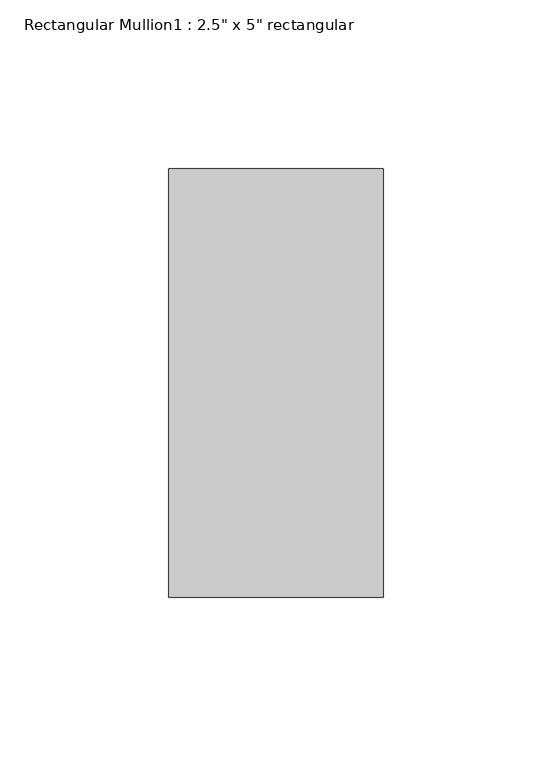
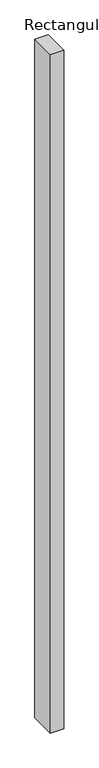
"""IFC4 building model written with IfcOpenShell, lengths in millimetres: member geometry."""

import ifcopenshell
import ifcopenshell.guid

model = None  # the IFC model being written
_history = None  # IfcOwnerHistory: only IFC2X3 demands one
_inside = {}  # id of a spatial element -> (the spatial element, [elements in it])
_under = {}  # id of a project, library or spatial element -> (it, [spatial elements below it])
_declared = {}  # id of a project -> (the project, [libraries it declares])
_typed = {}  # id of a type object -> (the type object, [elements of that type])
_made_of = {}  # id of a material, layer set ... -> (it, [elements and type objects made of it])


def new_model(schema):
    """Start an empty IFC model of exactly this schema.

    Asked for "IFC4X3", IfcOpenShell would pick the latest addendum, in which some entities
    have other attributes; the version numbers below select the first issue.
    IFC2X3 requires an IfcOwnerHistory on every rooted entity: one is made here for all.
    """
    global model, _history
    if schema == "IFC4X3":
        model = ifcopenshell.file(schema_version=(4, 3, 0, 0))
    else:
        model = ifcopenshell.file(schema=schema)
    _inside.clear()
    _under.clear()
    _declared.clear()
    _typed.clear()
    _made_of.clear()
    _history = None
    if model.schema == "IFC2X3":
        org = make("IfcOrganization", Name="unknown")
        user = make(
            "IfcPersonAndOrganization",
            ThePerson=make("IfcPerson", FamilyName="unknown"),
            TheOrganization=org,
        )
        app = make(
            "IfcApplication",
            ApplicationDeveloper=org,
            Version="unknown",
            ApplicationFullName="unknown",
            ApplicationIdentifier="unknown",
        )
        _history = make(
            "IfcOwnerHistory",
            OwningUser=user,
            OwningApplication=app,
            ChangeAction="ADDED",
            CreationDate=0,
        )
    return model


def make(cls, **values):
    """One entity of the class cls with the attributes given. An attribute that is None is left unset."""
    return model.create_entity(
        cls, **{name: value for name, value in values.items() if value is not None}
    )


def rooted(cls, **values):
    """An entity with a GlobalId (a new one), such as an element, a storey or a relation."""
    return make(cls, GlobalId=ifcopenshell.guid.new(), OwnerHistory=_history, **values)


def si_unit(unit_type, name, prefix=None):
    """IfcSIUnit, for example si_unit("LENGTHUNIT", "METRE", prefix="MILLI")."""
    return make("IfcSIUnit", UnitType=unit_type, Prefix=prefix, Name=name)


def assignment(units):
    """IfcUnitAssignment: the units of a project."""
    return None if units is None else make("IfcUnitAssignment", Units=units)


def point(xyz):
    """IfcCartesianPoint."""
    return None if xyz is None else make("IfcCartesianPoint", Coordinates=xyz)


def direction(xyz):
    """IfcDirection."""
    return None if xyz is None else make("IfcDirection", DirectionRatios=xyz)


def frame(location, z_axis=None, x_axis=None):
    """IfcAxis2Placement3D, a coordinate frame: its origin and axes. An axis left out is left unset."""
    return make(
        "IfcAxis2Placement3D",
        Location=point(location),
        Axis=direction(z_axis),
        RefDirection=direction(x_axis),
    )


def origin():
    """The frame at (0, 0, 0) with its axes left unset."""
    return frame((0.0, 0.0, 0.0))


def place(relative_to, where):
    """IfcLocalPlacement: puts the frame where relative to a parent placement (None: the world)."""
    return make(
        "IfcLocalPlacement", PlacementRelTo=relative_to, RelativePlacement=where
    )


def context(
    kind, dimensions, precision=None, world=None, true_north=None, identifier=None
):
    """IfcGeometricRepresentationContext, for example the 3D "Model" context."""
    return make(
        "IfcGeometricRepresentationContext",
        ContextIdentifier=identifier,
        ContextType=kind,
        CoordinateSpaceDimension=dimensions,
        Precision=precision,
        WorldCoordinateSystem=world,
        TrueNorth=true_north,
    )


def project(units=None, contexts=None):
    """IfcProject with its units and contexts."""
    return rooted(
        "IfcProject",
        Name="project",
        RepresentationContexts=contexts,
        UnitsInContext=assignment(units),
    )


def spatial(cls, under=None, at=None, **own):
    """A site, building, storey or space (cls), placed at a placement, below another one or the project."""
    s = rooted(cls, ObjectPlacement=at, **own)
    if under is not None:
        _under.setdefault(under.id(), (under, []))[1].append(s)
    return s


def polyline(points):
    """IfcPolyline through the points."""
    return make("IfcPolyline", Points=[point(p) for p in points])


def outline(outer, holes=None, kind="AREA"):
    """IfcArbitraryClosedProfileDef: a profile drawn as a closed curve; with holes, ...WithVoids."""
    if holes is None:
        return make("IfcArbitraryClosedProfileDef", ProfileType=kind, OuterCurve=outer)
    return make(
        "IfcArbitraryProfileDefWithVoids",
        ProfileType=kind,
        OuterCurve=outer,
        InnerCurves=holes,
    )


def extrude(swept, where, along, depth):
    """IfcExtrudedAreaSolid: the profile swept, set in the frame where, extruded along a direction by depth."""
    return make(
        "IfcExtrudedAreaSolid",
        SweptArea=swept,
        Position=where,
        ExtrudedDirection=direction(along),
        Depth=depth,
    )


def shape(context_of_items, identifier, shape_type, items):
    """IfcShapeRepresentation: the items that make up one representation, for example the "Body"."""
    return make(
        "IfcShapeRepresentation",
        ContextOfItems=context_of_items,
        RepresentationIdentifier=identifier,
        RepresentationType=shape_type,
        Items=items,
    )


def source(mapping_origin, context_of_items, identifier, shape_type, items):
    """IfcRepresentationMap: a shape defined once, which mapped items show again and again."""
    return make(
        "IfcRepresentationMap",
        MappingOrigin=mapping_origin,
        MappedRepresentation=shape(context_of_items, identifier, shape_type, items),
    )


def transform(
    local_origin,
    x_axis=None,
    y_axis=None,
    z_axis=None,
    scale=None,
    scale2=None,
    scale3=None,
    uniform=True,
):
    """IfcCartesianTransformationOperator3D, or its non-uniform kind. x_axis, y_axis, z_axis: its Axis1, 2, 3."""
    if uniform:
        return make(
            "IfcCartesianTransformationOperator3D",
            Axis1=direction(x_axis),
            Axis2=direction(y_axis),
            LocalOrigin=point(local_origin),
            Scale=scale,
            Axis3=direction(z_axis),
        )
    return make(
        "IfcCartesianTransformationOperator3DnonUniform",
        Axis1=direction(x_axis),
        Axis2=direction(y_axis),
        LocalOrigin=point(local_origin),
        Scale=scale,
        Axis3=direction(z_axis),
        Scale2=scale2,
        Scale3=scale3,
    )


def mapped(mapping_source, mapping_target):
    """IfcMappedItem: shows the shape of a source again, moved by a transform."""
    return make(
        "IfcMappedItem", MappingSource=mapping_source, MappingTarget=mapping_target
    )


def made_of(thing, what):
    """Note that an element or type object is made of a material, layer set ...; save() writes the relation."""
    if what is not None:
        _made_of.setdefault(what.id(), (what, []))[1].append(thing)
    return thing


def element(
    cls,
    number,
    at=None,
    inside=None,
    cuts=None,
    type_object=None,
    material=None,
    context=None,
    identifier="Body",
    shape_type=None,
    held_by="IfcProductDefinitionShape",
    body=None,
    shapes=None,
    **own,
):
    """One element of the class cls, such as IfcWall. Its Tag is "e" and its number.

    at: its placement. inside: the storey or other place that contains it. cuts: it is an
    opening in that element (IfcRelVoidsElement). A single representation is given by context,
    identifier, shape_type and body (its items); several are given by shapes. held_by: the class
    of the entity that holds the representations. save() writes the other relations.
    """
    e = rooted(cls, Tag="e%d" % number, ObjectPlacement=at, **own)
    if body is not None:
        shapes = [shape(context, identifier, shape_type, body)]
    if shapes is not None:
        e.Representation = make(held_by, Representations=shapes)
    if inside is not None:
        _inside.setdefault(inside.id(), (inside, []))[1].append(e)
    if cuts is not None:
        rooted(
            "IfcRelVoidsElement", RelatingBuildingElement=cuts, RelatedOpeningElement=e
        )
    if type_object is not None:
        _typed.setdefault(type_object.id(), (type_object, []))[1].append(e)
    return made_of(e, material)


def aggregate(whole, parts):
    """IfcRelAggregates: a whole, such as a stair, and the parts it consists of."""
    return rooted("IfcRelAggregates", RelatingObject=whole, RelatedObjects=parts)


def save(model, path):
    """Write the relations noted so far, then the file.

    IfcRelAggregates (storeys below a building ...), IfcRelContainedInSpatialStructure (elements
    in a storey), IfcRelDefinesByType, IfcRelAssociatesMaterial and IfcRelDeclares: one each for
    every whole, place, type object, material and project.
    """
    for whole, parts in _under.values():
        aggregate(whole, parts)
    for where, things in _inside.values():
        rooted(
            "IfcRelContainedInSpatialStructure",
            RelatedElements=things,
            RelatingStructure=where,
        )
    for kind, things in _typed.values():
        rooted("IfcRelDefinesByType", RelatedObjects=things, RelatingType=kind)
    for what, things in _made_of.values():
        rooted("IfcRelAssociatesMaterial", RelatedObjects=things, RelatingMaterial=what)
    for by, libraries in _declared.values():
        rooted("IfcRelDeclares", RelatingContext=by, RelatedDefinitions=libraries)
    model.write(path)


def member_7b18d258(model_context):
    return source(origin(), model_context, "Body", "SweptSolid", [
        extrude(outline(polyline([(31.75, 63.5), (31.75, -63.5), (-31.75, -63.5), (-31.75, 63.5), (31.75, 63.5)])), frame((0.0, 0.0, -3382.4333333), z_axis=(0.0, 0.0, 1.0), x_axis=(1.0, 0.0, 0.0)), (0.0, 0.0, 1.0), 3382.4333333),
    ])


if __name__ == "__main__":
    model = new_model("IFC4")
    model_context = context("Model", 3, world=origin())
    ifc_project = project(units=[si_unit("LENGTHUNIT", "METRE", prefix="MILLI")], contexts=[model_context])
    site = spatial("IfcSite", under=ifc_project)
    building = spatial("IfcBuilding", under=site)
    placement = place(None, origin())
    member_shape = member_7b18d258(model_context)
    element("IfcMember", 1, ObjectType="Rectangular Mullion1 : 2.5\" x 5\" rectangular", at=placement, inside=building, context=model_context, shape_type="MappedRepresentation", body=[
        mapped(member_shape, transform((0.0, 0.0, 0.0), x_axis=(1.0, 0.0, 0.0), y_axis=(0.0, 1.0, 0.0), z_axis=(0.0, 0.0, 1.0))),
    ])
    save(model, "model.ifc")

# Revit data of these elements
# Type "Rectangular Mullion1 : 2.5\" x 5\" rectangular"
#   built-in parameter 1007304 = 0.416667 (stored number, unit not read)
#   built-in parameter 1007301 = 0.104167 (stored number, unit not read)
#   built-in parameter 1007300 = 0.104167 (stored number, unit not read)
# Element 1 (IfcMember, "Rectangular Mullion1 : 2.5\" x 5\" rectangular")
#   Materials on its faces: "support-frame"
# Materials
#   "support-frame": class "Unassigned", colour RGB 233 233 233, transparency 0, Cost = 0
